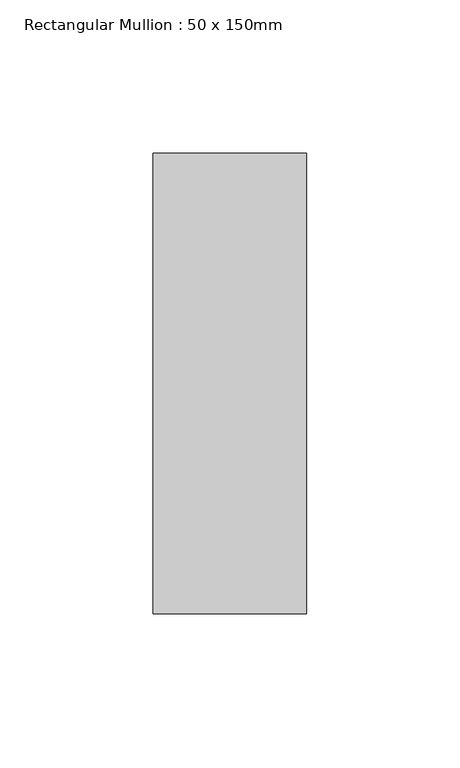
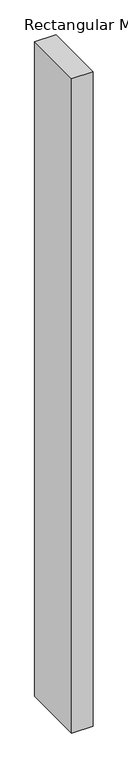
"""IFC4 building model written with IfcOpenShell, lengths in millimetres: member geometry, Rectangular Mullion : 50 x 150mm."""

from ifc_helpers import new_model, si_unit, frame, origin, place, context, project, spatial, polyline, outline, extrude, source, transform, mapped, element, save


def rectangular_mullion_50_x_150mm_128e4daa(model_context):
    return source(origin(), model_context, "Body", "SweptSolid", [
        extrude(outline(polyline([(0.0, 75.0), (0.0, -75.0), (-50.0, -75.0), (-50.0, 75.0), (0.0, 75.0)])), frame((0.0, 0.0, -1615.55), z_axis=(0.0, 0.0, 1.0), x_axis=(1.0, 0.0, 0.0)), (0.0, 0.0, 1.0), 1615.55),
    ])


if __name__ == "__main__":
    model = new_model("IFC4")
    model_context = context("Model", 3, world=origin())
    ifc_project = project(units=[si_unit("LENGTHUNIT", "METRE", prefix="MILLI")], contexts=[model_context])
    site = spatial("IfcSite", under=ifc_project)
    building = spatial("IfcBuilding", under=site)
    placement = place(None, origin())
    rectangular_mullion_50_x_150mm_shape = rectangular_mullion_50_x_150mm_128e4daa(model_context)
    element("IfcMember", 1, ObjectType="Rectangular Mullion : 50 x 150mm", at=placement, inside=building, context=model_context, shape_type="MappedRepresentation", body=[
        mapped(rectangular_mullion_50_x_150mm_shape, transform((0.0, 0.0, 0.0), x_axis=(1.0, 0.0, 0.0), y_axis=(0.0, 1.0, 0.0), z_axis=(0.0, 0.0, 1.0))),
    ])
    save(model, "model.ifc")

# Revit data of these elements
# Type "Rectangular Mullion : 50 x 150mm"
#   Keynote = "H11"
#   built-in parameter 1007304 = 0.492126 (stored number, unit not read)
#   built-in parameter 1007301 = 0.082021 (stored number, unit not read)
#   built-in parameter 1007300 = 0.082021 (stored number, unit not read)
# Element 1 (IfcMember, "Rectangular Mullion : 50 x 150mm")
#   Materials on its faces: "Aluminium"
# Materials
#   "Aluminium": class "Metal", colour RGB 247 247 247, transparency 0, Description = "Aluminium 6061", Cost = 0
